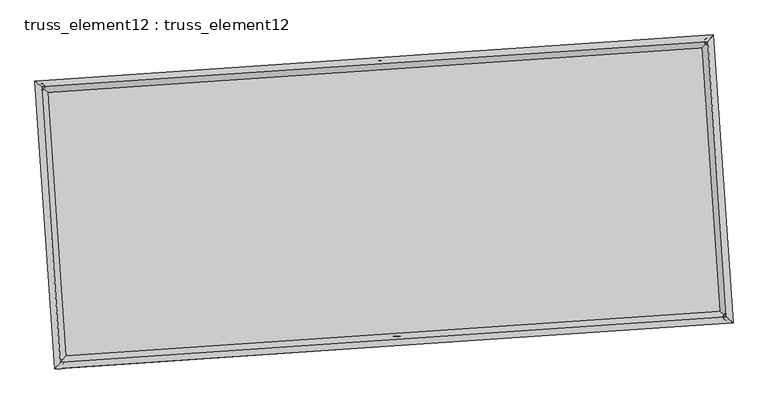
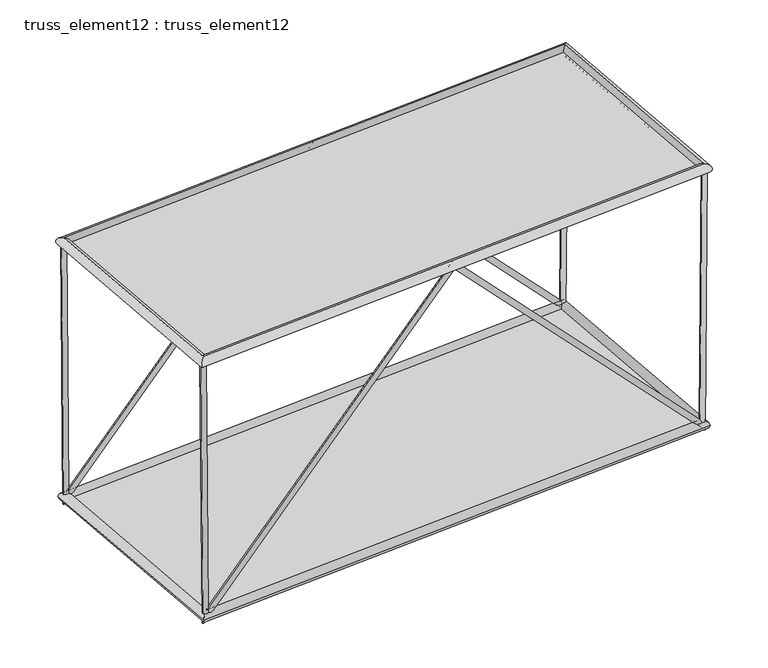
"""IFC4 building model written with IfcOpenShell, lengths in millimetres: plate geometry, truss_element12 : truss_element12."""

from ifc_helpers import new_model, si_unit, frame, origin, origin_with_axes, place, context, project, spatial, polyline, circle_curve, ellipse_curve, outline, extrude, source, transform, mapped, element, save
from ifc_brep_helpers import plane_surface, cylinder_surface, advanced_brep


def truss_element12_truss_element12_50c5f4de(model_context):
    return source(origin(), model_context, "Body", "SolidModel", [
        advanced_brep(
        [(-3706.5799922, 2273.384825, 5000.2422562), (-3805.6798862, 2260.0237861, 4999.4094062), (-3665.9654845, 2276.1541738, 123.1398284), (-3763.0213983, 2262.9325063, -123.1398284), (1063.3743775, 2598.6298811, 5071.9513391), (1063.8277335, 2592.057, 4927.7060065), (5793.3875538, 2921.1514992, 123.1446756), (5891.3734232, 2921.2289893, -123.1446756), (5833.3338428, 2923.8752848, 5000.2410891), (5933.3302575, 2924.0898664, 4999.4219398)],
        [
            (0, 1, circle_curve(frame((-3756.1299392, 2266.7043055, 4999.8258312), z_axis=(-0.008327299552923583, -0.0005678069014846499, 0.9999651662320437), x_axis=(-0.13361046312996155, 0.9910337742643954, -0.0005499176889615099)), 50.0)),
            (1, 0, circle_curve(frame((-3756.1299392, 2266.7043055, 4999.8258312), z_axis=(-0.008327299552923583, -0.0005678069014846499, 0.9999651662320437), x_axis=(-0.13361046312996155, 0.9910337742643954, -0.0005499176889615099)), 50.0)),
            (0, 2),
            (2, 3, ellipse_curve(frame((-3714.4934414, 2269.54334, 0.0), z_axis=(-0.9273368066437185, -0.06323157170781193, 0.36884714365600024), x_axis=(0.36799267091523613, 0.025092021358606446, 0.9294900669812509)), 132.7695372, 50.0)),
            (3, 1),
            (3, 2, ellipse_curve(frame((-3714.4934414, 2269.54334, 0.0), z_axis=(-0.9273368066437185, -0.06323157170781193, 0.36884714365600024), x_axis=(0.36799267091523613, 0.025092021358606446, 0.9294900669812509)), 132.7695372, 50.0)),
            (2, 4),
            (4, 5, ellipse_curve(frame((1063.6010555, 2595.3434406, 4999.8286728), z_axis=(-0.9976833954354812, -0.06802823818510302, -3.58016770651758e-05), x_axis=(3.571873875964661e-05, 2.435525016045128e-06, -0.99999999935912)), 72.2797139, 50.0)),
            (5, 3),
            (5, 4, ellipse_curve(frame((1063.6010555, 2595.3434406, 4999.8286728), z_axis=(-0.9976833954354812, -0.06802823818510302, -3.58016770651758e-05), x_axis=(3.571873875964661e-05, 2.435525016045128e-06, -0.99999999935912)), 72.2797139, 50.0)),
            (4, 6),
            (6, 7, ellipse_curve(frame((5842.3804885, 2921.1902443, 0.0), z_axis=(-0.9272983622915061, -0.06322895033357485, -0.3689442330911339), x_axis=(-0.3680895354326035, -0.02509862618182887, 0.9294515333619042)), 132.780268, 50.0)),
            (7, 5),
            (7, 6, ellipse_curve(frame((5842.3804885, 2921.1902443, 0.0), z_axis=(-0.9272983622915061, -0.06322895033357485, -0.3689442330911339), x_axis=(-0.3680895354326035, -0.02509862618182887, 0.9294515333619042)), 132.780268, 50.0)),
            (8, 9, circle_curve(frame((5883.3320502, 2923.9825756, 4999.8315144), z_axis=(0.008190312331474266, 0.0005584662635913799, 0.9999663028819249), x_axis=(-0.0021503186312376984, 0.99999754179097, -0.0005408713353677941)), 50.0)),
            (9, 8, circle_curve(frame((5883.3320502, 2923.9825756, 4999.8315144), z_axis=(0.008190312331474266, 0.0005584662635913799, 0.9999663028819249), x_axis=(-0.0021503186312376984, 0.99999754179097, -0.0005408713353677941)), 50.0)),
            (6, 8),
            (9, 7),
        ],
        [
            plane_surface(frame((-3756.1299392, 2316.7042975, 4999.8542225), z_axis=(-0.008327299552923011, -0.0005678069014865664, 0.9999651662320436), x_axis=(0.9999653274399848, -4.72846210453071e-06, 0.008327298210449648))),
            cylinder_surface(frame((-3756.1299392, 2266.7043055, 4999.8258312), z_axis=(-0.008327299552923583, -0.0005678069014846499, 0.9999651662320437), x_axis=(-0.13361046312996155, 0.9910337742643954, -0.0005499176889615099)), 50.0),
            cylinder_surface(frame((-3714.4934414, 2269.54334, 0.0), z_axis=(-0.6901287062724669, -0.04705725305590364, -0.7221550967164351), x_axis=(-0.020411495011476707, 0.9987523815908318, -0.0455746764995446)), 50.0),
            cylinder_surface(frame((1063.6010555, 2595.3434406, 4999.8286728), z_axis=(-0.6901802934417622, -0.04706077058887624, 0.7221055645930341), x_axis=(-0.11534610560274808, 0.9922791513748532, -0.045578083209815906)), 50.0),
            plane_surface(frame((5883.3320502, 2873.9825834, 4999.8594387), z_axis=(0.008190312331473465, 0.0005584662635926667, 0.9999663028819249), x_axis=(0.9999664588294515, -4.574166547754999e-06, -0.008190311054171673))),
            cylinder_surface(frame((5842.3804885, 2921.1902443, 0.0), z_axis=(-0.008190312331474266, -0.0005584662635913799, -0.9999663028819249), x_axis=(-0.0021503186312376984, 0.99999754179097, -0.0005408713353677941)), 50.0),
        ],
        [
            (0, [[1, 2]]),
            (1, [[-1, 3, 4, 5]]),
            (1, [[-2, -5, 6, -3]]),
            (2, [[-4, 7, 8, 9]]),
            (2, [[-6, -9, 10, -7]]),
            (3, [[-8, 11, 12, 13]]),
            (3, [[-10, -13, 14, -11]]),
            (4, [[15, 16]]),
            (5, [[-12, 17, -16, 18]]),
            (5, [[-14, -18, -15, -17]]),
        ],
    ),
        advanced_brep(
        [(-3434.4670392, -1717.3487593, 5000.2422562), (-3533.5669333, -1730.7097982, 4999.4094062), (-3393.8525316, -1714.5794105, 123.1398284), (-3490.9084454, -1727.801078, -123.1398284), (1335.4873304, -1392.1037032, 5071.9513391), (1335.9406864, -1398.6765843, 4927.7060065), (6065.5005068, -1069.5820851, 123.1446756), (6163.4863761, -1069.504595, -123.1446756), (6105.4467957, -1066.8582995, 5000.2410891), (6205.4432104, -1066.6437179, 4999.4219398)],
        [
            (0, 1, circle_curve(frame((-3484.0169863, -1724.0292788, 4999.8258312), z_axis=(-0.008327299552923084, -0.0005678069014846462, 0.9999651662320437), x_axis=(-0.13361046312996083, 0.9910337742643955, -0.0005499176889614408)), 50.0)),
            (1, 0, circle_curve(frame((-3484.0169863, -1724.0292788, 4999.8258312), z_axis=(-0.008327299552923084, -0.0005678069014846462, 0.9999651662320437), x_axis=(-0.13361046312996083, 0.9910337742643955, -0.0005499176889614408)), 50.0)),
            (0, 2),
            (2, 3, ellipse_curve(frame((-3442.3804885, -1721.1902443, 0.0), z_axis=(-0.9273368066437186, -0.06323157170781156, 0.36884714365600035), x_axis=(0.3679926709152363, 0.02509202135860627, 0.9294900669812506)), 132.7695372, 50.0)),
            (3, 1),
            (3, 2, ellipse_curve(frame((-3442.3804885, -1721.1902443, 0.0), z_axis=(-0.9273368066437186, -0.06323157170781156, 0.36884714365600035), x_axis=(0.3679926709152363, 0.02509202135860627, 0.9294900669812506)), 132.7695372, 50.0)),
            (2, 4),
            (4, 5, ellipse_curve(frame((1335.7140084, -1395.3901437, 4999.8286728), z_axis=(-0.9976833954354812, -0.06802823818510288, -3.58016770651758e-05), x_axis=(3.571873875964661e-05, 2.435525016352613e-06, -0.99999999935912)), 72.2797139, 50.0)),
            (5, 3),
            (5, 4, ellipse_curve(frame((1335.7140084, -1395.3901437, 4999.8286728), z_axis=(-0.9976833954354812, -0.06802823818510288, -3.58016770651758e-05), x_axis=(3.571873875964661e-05, 2.435525016352613e-06, -0.99999999935912)), 72.2797139, 50.0)),
            (4, 6),
            (6, 7, ellipse_curve(frame((6114.4934414, -1069.54334, 0.0), z_axis=(-0.9272983622915062, -0.06322895033357505, -0.3689442330911336), x_axis=(-0.3680895354326032, -0.0250986261818289, 0.9294515333619043)), 132.780268, 50.0)),
            (7, 5),
            (7, 6, ellipse_curve(frame((6114.4934414, -1069.54334, 0.0), z_axis=(-0.9272983622915062, -0.06322895033357505, -0.3689442330911336), x_axis=(-0.3680895354326032, -0.0250986261818289, 0.9294515333619043)), 132.780268, 50.0)),
            (8, 9, circle_curve(frame((6155.4450031, -1066.7510087, 4999.8315144), z_axis=(0.008190312331474381, 0.0005584662635914046, 0.9999663028819248), x_axis=(-0.0021503186312381295, 0.99999754179097, -0.0005408713353678152)), 50.0)),
            (9, 8, circle_curve(frame((6155.4450031, -1066.7510087, 4999.8315144), z_axis=(0.008190312331474381, 0.0005584662635914046, 0.9999663028819248), x_axis=(-0.0021503186312381295, 0.99999754179097, -0.0005408713353678152)), 50.0)),
            (6, 8),
            (9, 7),
        ],
        [
            plane_surface(frame((-3484.0169863, -1674.0292868, 4999.8542225), z_axis=(-0.008327299552923011, -0.0005678069014865726, 0.9999651662320436), x_axis=(0.9999653274399848, -4.72846210453071e-06, 0.008327298210449648))),
            cylinder_surface(frame((-3484.0169863, -1724.0292788, 4999.8258312), z_axis=(-0.008327299552923084, -0.0005678069014846462, 0.9999651662320437), x_axis=(-0.13361046312996083, 0.9910337742643955, -0.0005499176889614408)), 50.0),
            cylinder_surface(frame((-3442.3804885, -1721.1902443, 0.0), z_axis=(-0.6901287062724669, -0.047057253055903324, -0.7221550967164352), x_axis=(-0.020411495011476505, 0.9987523815908318, -0.045574676499544345)), 50.0),
            cylinder_surface(frame((1335.7140084, -1395.3901437, 4999.8286728), z_axis=(-0.690180293441762, -0.04706077058887634, 0.722105564593034), x_axis=(-0.11534610560274797, 0.9922791513748532, -0.045578083209815635)), 50.0),
            plane_surface(frame((6155.4450031, -1116.7510009, 4999.8594387), z_axis=(0.008190312331473467, 0.000558466263592672, 0.9999663028819249), x_axis=(0.9999664588294515, -4.574166548199088e-06, -0.008190311054171673))),
            cylinder_surface(frame((6114.4934414, -1069.54334, 0.0), z_axis=(-0.008190312331474381, -0.0005584662635914046, -0.9999663028819248), x_axis=(-0.0021503186312381295, 0.99999754179097, -0.0005408713353678152)), 50.0),
        ],
        [
            (0, [[1, 2]]),
            (1, [[-1, 3, 4, 5]]),
            (1, [[-2, -5, 6, -3]]),
            (2, [[-4, 7, 8, 9]]),
            (2, [[-6, -9, 10, -7]]),
            (3, [[-8, 11, 12, 13]]),
            (3, [[-10, -13, 14, -11]]),
            (4, [[15, 16]]),
            (5, [[-12, 17, -16, 18]]),
            (5, [[-14, -18, -15, -17]]),
        ],
    ),
        advanced_brep(
        [(-3484.0154882, -1724.0276184, 4909.8258312), (-3484.0184843, -1724.0309391, 5089.8258311), (-3756.1316487, 2266.7057472, 5089.8258311), (-3756.1282296, 2266.7028639, 4909.8258312), (5883.3334426, 2923.9842287, 5089.8315144), (5883.3306577, 2923.9809224, 4909.8315144), (6155.446607, -1066.7524576, 5089.8315144), (6155.4433991, -1066.7495599, 4909.8315144)],
        [
            (0, 1, ellipse_curve(frame((-3484.0169863, -1724.0292788, 4999.8258312), z_axis=(-0.7535719234053359, 0.6573654662780891, -4.159313612812967e-07), x_axis=(-0.6573654662779587, -0.7535719234054498, -4.1593136128130245e-07)), 127.2792206, 90.0)),
            (1, 2),
            (2, 3, ellipse_curve(frame((-3756.1299392, 2266.7043055, 4999.8258312), z_axis=(-0.6573654662779587, -0.7535719234054498, -4.1593136128130664e-07), x_axis=(0.753571923405336, -0.657365466278089, 4.1593136128130097e-07)), 127.2792206, 90.0)),
            (3, 0),
            (1, 0, ellipse_curve(frame((-3484.0169863, -1724.0292788, 4999.8258312), z_axis=(-0.7535719234053359, 0.6573654662780891, -4.159313612812967e-07), x_axis=(-0.6573654662779587, -0.7535719234054498, -4.1593136128130245e-07)), 127.2792206, 90.0)),
            (3, 2, ellipse_curve(frame((-3756.1299392, 2266.7043055, 4999.8258312), z_axis=(-0.6573654662779587, -0.7535719234054498, -4.1593136128130664e-07), x_axis=(0.753571923405336, -0.657365466278089, 4.1593136128130097e-07)), 127.2792206, 90.0)),
            (2, 4),
            (4, 5, ellipse_curve(frame((5883.3320502, 2923.9825756, 4999.8315144), z_axis=(-0.7535719234053357, 0.6573654662780891, -4.159313612813051e-07), x_axis=(-0.6573654662779591, -0.7535719234054494, -4.159313612813025e-07)), 127.2792206, 90.0)),
            (5, 3),
            (5, 4, ellipse_curve(frame((5883.3320502, 2923.9825756, 4999.8315144), z_axis=(-0.7535719234053357, 0.6573654662780891, -4.159313612813051e-07), x_axis=(-0.6573654662779591, -0.7535719234054494, -4.159313612813025e-07)), 127.2792206, 90.0)),
            (4, 6),
            (6, 7, ellipse_curve(frame((6155.4450031, -1066.7510087, 4999.8315144), z_axis=(0.6573654662779589, 0.7535719234054495, 4.1593136128129817e-07), x_axis=(-0.7535719234053357, 0.6573654662780891, -4.159313612813009e-07)), 127.2792206, 90.0)),
            (7, 5),
            (7, 6, ellipse_curve(frame((6155.4450031, -1066.7510087, 4999.8315144), z_axis=(0.6573654662779589, 0.7535719234054495, 4.1593136128129817e-07), x_axis=(-0.7535719234053357, 0.6573654662780891, -4.159313612813009e-07)), 127.2792206, 90.0)),
            (6, 1),
            (0, 7),
        ],
        [
            cylinder_surface(frame((-3484.0169863, -1724.0292788, 4999.8258312), z_axis=(0.06802823822870238, -0.9976833960748767, 0.0), x_axis=(-0.9976833959157302, -0.06802823821785078, -1.786146746609056e-05)), 90.0),
            cylinder_surface(frame((-3756.1299392, 2266.7043055, 4999.8258312), z_axis=(-0.9976833960747041, -0.06802823822868846, -5.882157721403235e-07), x_axis=(-0.06802823820841473, 0.9976833959267308, -1.7273251694037993e-05)), 90.0),
            cylinder_surface(frame((5883.3320502, 2923.9825756, 4999.8315144), z_axis=(-0.06802823822870215, 0.9976833960748767, 0.0), x_axis=(0.9976833959360039, 0.06802823821923294, -1.6685035921985425e-05)), 90.0),
            cylinder_surface(frame((6155.4450031, -1066.7510087, 4999.8315144), z_axis=(0.997683396074704, 0.06802823822868831, 5.882157721403174e-07), x_axis=(0.06802823822868831, -0.9976833959253485, -1.7273251694037996e-05)), 90.0),
        ],
        [
            (0, [[1, 2, 3, 4]]),
            (0, [[5, -4, 6, -2]]),
            (1, [[-3, 7, 8, 9]]),
            (1, [[-6, -9, 10, -7]]),
            (2, [[-8, 11, 12, 13]]),
            (2, [[-10, -13, 14, -11]]),
            (3, [[-12, 15, -1, 16]]),
            (3, [[-14, -16, -5, -15]]),
        ],
    ),
        advanced_brep(
        [(-3358.7115243, -1625.2761972, 0.0), (-3526.0494527, -1817.1042913, 0.0), (-3810.4074885, 2353.2123043, 0.0), (-3618.5793943, 2185.8743758, 0.0), (5926.0494527, 3017.1042913, 0.0), (5758.7115243, 2825.2761972, 0.0), (6210.4074885, -1153.2123043, 0.0), (6018.5793943, -985.8743758, 0.0)],
        [
            (0, 1, ellipse_curve(frame((-3442.3804885, -1721.1902443, 0.0), z_axis=(-0.7535719234054581, 0.6573654662780806, 0.0), x_axis=(-0.6573654662780807, -0.7535719234054581, 0.0)), 127.2792206, 90.0)),
            (1, 2),
            (2, 3, ellipse_curve(frame((-3714.4934414, 2269.54334, 0.0), z_axis=(-0.6573654662780806, -0.7535719234054582, 0.0), x_axis=(0.7535719234054581, -0.6573654662780805, 0.0)), 127.2792206, 90.0)),
            (3, 0),
            (1, 0, ellipse_curve(frame((-3442.3804885, -1721.1902443, 0.0), z_axis=(-0.7535719234054581, 0.6573654662780806, 0.0), x_axis=(-0.6573654662780807, -0.7535719234054581, 0.0)), 127.2792206, 90.0)),
            (3, 2, ellipse_curve(frame((-3714.4934414, 2269.54334, 0.0), z_axis=(-0.6573654662780806, -0.7535719234054582, 0.0), x_axis=(0.7535719234054581, -0.6573654662780805, 0.0)), 127.2792206, 90.0)),
            (2, 4),
            (4, 5, ellipse_curve(frame((5842.3804885, 2921.1902443, 0.0), z_axis=(-0.7535719234054581, 0.6573654662780806, 0.0), x_axis=(-0.6573654662780808, -0.7535719234054579, 0.0)), 127.2792206, 90.0)),
            (5, 3),
            (5, 4, ellipse_curve(frame((5842.3804885, 2921.1902443, 0.0), z_axis=(-0.7535719234054581, 0.6573654662780806, 0.0), x_axis=(-0.6573654662780808, -0.7535719234054579, 0.0)), 127.2792206, 90.0)),
            (4, 6),
            (6, 7, ellipse_curve(frame((6114.4934414, -1069.54334, 0.0), z_axis=(0.6573654662780807, 0.753571923405458, 0.0), x_axis=(-0.7535719234054581, 0.6573654662780807, 0.0)), 127.2792206, 90.0)),
            (7, 5),
            (7, 6, ellipse_curve(frame((6114.4934414, -1069.54334, 0.0), z_axis=(0.6573654662780807, 0.753571923405458, 0.0), x_axis=(-0.7535719234054581, 0.6573654662780807, 0.0)), 127.2792206, 90.0)),
            (6, 1),
            (0, 7),
        ],
        [
            cylinder_surface(frame((-3442.3804885, -1721.1902443, 0.0), z_axis=(0.0680282382287027, -0.9976833960748764, 0.0), x_axis=(-0.9976833960748764, -0.0680282382287027, 0.0)), 90.0),
            cylinder_surface(frame((-3714.4934414, 2269.54334, 0.0), z_axis=(-0.9976833960748767, -0.0680282382287005, 0.0), x_axis=(-0.0680282382287005, 0.9976833960748767, 0.0)), 90.0),
            cylinder_surface(frame((5842.3804885, 2921.1902443, 0.0), z_axis=(-0.06802823822870246, 0.9976833960748765, 0.0), x_axis=(0.9976833960748765, 0.06802823822870246, 0.0)), 90.0),
            cylinder_surface(frame((6114.4934414, -1069.54334, 0.0), z_axis=(0.9976833960748767, 0.06802823822870033, 0.0), x_axis=(0.06802823822870033, -0.9976833960748767, 0.0)), 90.0),
        ],
        [
            (0, [[1, 2, 3, 4]]),
            (0, [[5, -4, 6, -2]]),
            (1, [[-3, 7, 8, 9]]),
            (1, [[-6, -9, 10, -7]]),
            (2, [[-8, 11, 12, 13]]),
            (2, [[-10, -13, 14, -11]]),
            (3, [[-12, 15, -1, 16]]),
            (3, [[-14, -16, -5, -15]]),
        ],
    ),
        extrude(outline(polyline([(-3442.3804885, -1721.1902443), (-3714.4934414, 2269.54334), (5842.3804885, 2921.1902443), (6114.4934414, -1069.54334), (-3442.3804885, -1721.1902443)])), origin_with_axes(), (0.0, 0.0, 1.0), 20.0),
        extrude(outline(polyline([(-2000.0, 4830.9223283), (2000.0, 4830.9223283), (2000.0, -4830.9223284), (-2000.0, -4830.9223284), (-2000.0, 4830.9223283)])), frame((1199.6575319, 599.9766484, 4999.8286728), z_axis=(-5.868531091737606e-07, -4.0015282677042145e-08, 0.999999999999827), x_axis=(-0.06802823822870291, 0.9976833960748764, 0.0)), (0.0, 0.0, 1.0), 20.0),
    ])


if __name__ == "__main__":
    model = new_model("IFC4")
    model_context = context("Model", 3, world=origin())
    ifc_project = project(units=[si_unit("LENGTHUNIT", "METRE", prefix="MILLI")], contexts=[model_context])
    site = spatial("IfcSite", under=ifc_project)
    building = spatial("IfcBuilding", under=site)
    placement = place(None, origin())
    truss_element12_truss_element12_shape = truss_element12_truss_element12_50c5f4de(model_context)
    element("IfcPlate", 1, ObjectType="truss_element12 : truss_element12", at=placement, inside=building, context=model_context, shape_type="MappedRepresentation", body=[
        mapped(truss_element12_truss_element12_shape, transform((0.0, 0.0, 0.0), x_axis=(1.0, 0.0, 0.0), y_axis=(0.0, 1.0, 0.0), z_axis=(0.0, 0.0, 1.0))),
    ])
    save(model, "model.ifc")

# Revit data of these elements
# Type "truss_element12 : truss_element12"
#   steellbar1 = 90 mm
#   steelbar2 = 50 mm
#   offset1 = 5000 mm
#   M = Default Roof
# Element 1 (IfcPlate, "truss_element12 : truss_element12")
#   Materials on its faces: "Default Roof"
# Materials
#   "Default Roof": class "Miscellaneous", colour RGB 0 127 0, transparency 0, Comments = "Rendering appearance not upgraded Rendering appearance not upgraded ", Cost = 0
